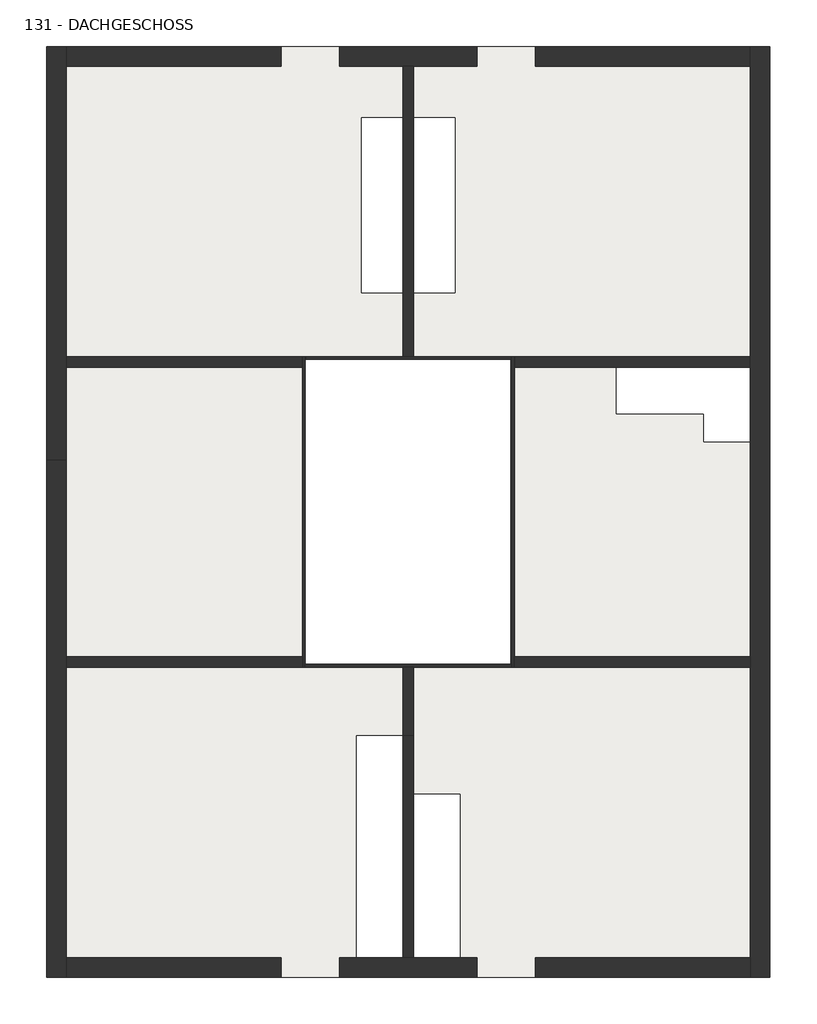
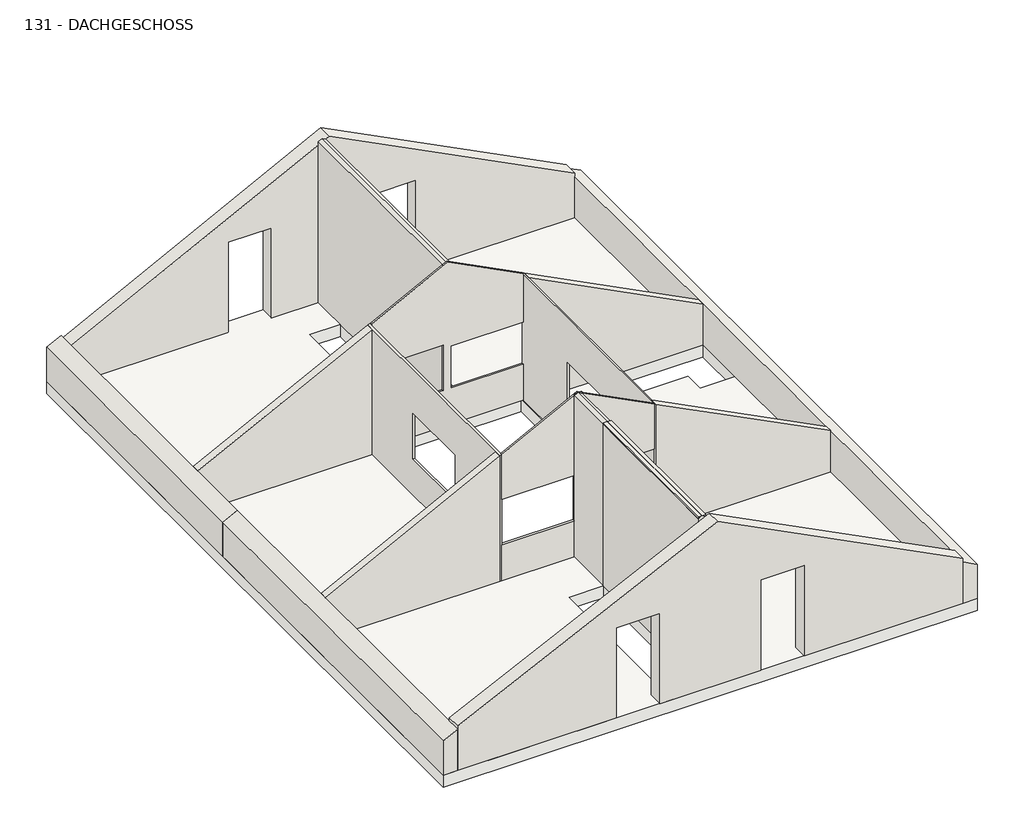
# One storey: 16 walls, 1 slab.
"""IFC4 building model written with IfcOpenShell, lengths in millimetres."""

import ifcopenshell
import ifcopenshell.guid

model = None  # the IFC model being written
_history = None  # IfcOwnerHistory: only IFC2X3 demands one
_inside = {}  # id of a spatial element -> (the spatial element, [elements in it])
_under = {}  # id of a project, library or spatial element -> (it, [spatial elements below it])
_declared = {}  # id of a project -> (the project, [libraries it declares])
_typed = {}  # id of a type object -> (the type object, [elements of that type])
_made_of = {}  # id of a material, layer set ... -> (it, [elements and type objects made of it])


def new_model(schema):
    """Start an empty IFC model of exactly this schema.

    Asked for "IFC4X3", IfcOpenShell would pick the latest addendum, in which some entities
    have other attributes; the version numbers below select the first issue.
    IFC2X3 requires an IfcOwnerHistory on every rooted entity: one is made here for all.
    """
    global model, _history
    if schema == "IFC4X3":
        model = ifcopenshell.file(schema_version=(4, 3, 0, 0))
    else:
        model = ifcopenshell.file(schema=schema)
    _inside.clear()
    _under.clear()
    _declared.clear()
    _typed.clear()
    _made_of.clear()
    _history = None
    if model.schema == "IFC2X3":
        org = make("IfcOrganization", Name="unknown")
        user = make(
            "IfcPersonAndOrganization",
            ThePerson=make("IfcPerson", FamilyName="unknown"),
            TheOrganization=org,
        )
        app = make(
            "IfcApplication",
            ApplicationDeveloper=org,
            Version="unknown",
            ApplicationFullName="unknown",
            ApplicationIdentifier="unknown",
        )
        _history = make(
            "IfcOwnerHistory",
            OwningUser=user,
            OwningApplication=app,
            ChangeAction="ADDED",
            CreationDate=0,
        )
    return model


def make(cls, **values):
    """One entity of the class cls with the attributes given. An attribute that is None is left unset."""
    return model.create_entity(
        cls, **{name: value for name, value in values.items() if value is not None}
    )


def rooted(cls, **values):
    """An entity with a GlobalId (a new one), such as an element, a storey or a relation."""
    return make(cls, GlobalId=ifcopenshell.guid.new(), OwnerHistory=_history, **values)


def si_unit(unit_type, name, prefix=None):
    """IfcSIUnit, for example si_unit("LENGTHUNIT", "METRE", prefix="MILLI")."""
    return make("IfcSIUnit", UnitType=unit_type, Prefix=prefix, Name=name)


def assignment(units):
    """IfcUnitAssignment: the units of a project."""
    return None if units is None else make("IfcUnitAssignment", Units=units)


def point(xyz):
    """IfcCartesianPoint."""
    return None if xyz is None else make("IfcCartesianPoint", Coordinates=xyz)


def direction(xyz):
    """IfcDirection."""
    return None if xyz is None else make("IfcDirection", DirectionRatios=xyz)


def frame(location, z_axis=None, x_axis=None):
    """IfcAxis2Placement3D, a coordinate frame: its origin and axes. An axis left out is left unset."""
    return make(
        "IfcAxis2Placement3D",
        Location=point(location),
        Axis=direction(z_axis),
        RefDirection=direction(x_axis),
    )


def origin():
    """The frame at (0, 0, 0) with its axes left unset."""
    return frame((0.0, 0.0, 0.0))


def place(relative_to, where):
    """IfcLocalPlacement: puts the frame where relative to a parent placement (None: the world)."""
    return make(
        "IfcLocalPlacement", PlacementRelTo=relative_to, RelativePlacement=where
    )


def context(
    kind, dimensions, precision=None, world=None, true_north=None, identifier=None
):
    """IfcGeometricRepresentationContext, for example the 3D "Model" context."""
    return make(
        "IfcGeometricRepresentationContext",
        ContextIdentifier=identifier,
        ContextType=kind,
        CoordinateSpaceDimension=dimensions,
        Precision=precision,
        WorldCoordinateSystem=world,
        TrueNorth=true_north,
    )


def project(units=None, contexts=None):
    """IfcProject with its units and contexts."""
    return rooted(
        "IfcProject",
        Name="project",
        RepresentationContexts=contexts,
        UnitsInContext=assignment(units),
    )


def spatial(cls, under=None, at=None, **own):
    """A site, building, storey or space (cls), placed at a placement, below another one or the project."""
    s = rooted(cls, ObjectPlacement=at, **own)
    if under is not None:
        _under.setdefault(under.id(), (under, []))[1].append(s)
    return s


def polyline(points):
    """IfcPolyline through the points."""
    return make("IfcPolyline", Points=[point(p) for p in points])


def outline(outer, holes=None, kind="AREA"):
    """IfcArbitraryClosedProfileDef: a profile drawn as a closed curve; with holes, ...WithVoids."""
    if holes is None:
        return make("IfcArbitraryClosedProfileDef", ProfileType=kind, OuterCurve=outer)
    return make(
        "IfcArbitraryProfileDefWithVoids",
        ProfileType=kind,
        OuterCurve=outer,
        InnerCurves=holes,
    )


def extrude(swept, where, along, depth):
    """IfcExtrudedAreaSolid: the profile swept, set in the frame where, extruded along a direction by depth."""
    return make(
        "IfcExtrudedAreaSolid",
        SweptArea=swept,
        Position=where,
        ExtrudedDirection=direction(along),
        Depth=depth,
    )


def faces_of(points, faces, orient=None, outer=None):
    """IfcFace entities. A face is a list of loops; a loop is a list of indices into points, from 0.

    orient and outer hold one flag for each loop. By default every Orientation is true, the
    first loop of a face is its IfcFaceOuterBound and the others are IfcFaceBound.
    """
    made = []
    for i, loops in enumerate(faces):
        bounds = []
        for j, loop in enumerate(loops):
            is_outer = j == 0 if outer is None else outer[i][j]
            bounds.append(
                make(
                    "IfcFaceOuterBound" if is_outer else "IfcFaceBound",
                    Bound=make("IfcPolyLoop", Polygon=[points[k] for k in loop]),
                    Orientation=True if orient is None else orient[i][j],
                )
            )
        made.append(make("IfcFace", Bounds=bounds))
    return made


def faceted_brep(points, faces, orient=None, outer=None, voids=None):
    """IfcFacetedBrep: a solid bounded by flat faces; with voids (closed shells), ...WithVoids."""
    shared = [point(p) for p in points]
    hull = make("IfcClosedShell", CfsFaces=faces_of(shared, faces, orient, outer))
    if voids is None:
        return make("IfcFacetedBrep", Outer=hull)
    return make(
        "IfcFacetedBrepWithVoids",
        Outer=hull,
        Voids=[
            make(cls, CfsFaces=faces_of(shared, fs, o, b)) for cls, fs, o, b in voids
        ],
    )


def shape(context_of_items, identifier, shape_type, items):
    """IfcShapeRepresentation: the items that make up one representation, for example the "Body"."""
    return make(
        "IfcShapeRepresentation",
        ContextOfItems=context_of_items,
        RepresentationIdentifier=identifier,
        RepresentationType=shape_type,
        Items=items,
    )


def source(mapping_origin, context_of_items, identifier, shape_type, items):
    """IfcRepresentationMap: a shape defined once, which mapped items show again and again."""
    return make(
        "IfcRepresentationMap",
        MappingOrigin=mapping_origin,
        MappedRepresentation=shape(context_of_items, identifier, shape_type, items),
    )


def transform(
    local_origin,
    x_axis=None,
    y_axis=None,
    z_axis=None,
    scale=None,
    scale2=None,
    scale3=None,
    uniform=True,
):
    """IfcCartesianTransformationOperator3D, or its non-uniform kind. x_axis, y_axis, z_axis: its Axis1, 2, 3."""
    if uniform:
        return make(
            "IfcCartesianTransformationOperator3D",
            Axis1=direction(x_axis),
            Axis2=direction(y_axis),
            LocalOrigin=point(local_origin),
            Scale=scale,
            Axis3=direction(z_axis),
        )
    return make(
        "IfcCartesianTransformationOperator3DnonUniform",
        Axis1=direction(x_axis),
        Axis2=direction(y_axis),
        LocalOrigin=point(local_origin),
        Scale=scale,
        Axis3=direction(z_axis),
        Scale2=scale2,
        Scale3=scale3,
    )


def mapped(mapping_source, mapping_target):
    """IfcMappedItem: shows the shape of a source again, moved by a transform."""
    return make(
        "IfcMappedItem", MappingSource=mapping_source, MappingTarget=mapping_target
    )


def made_of(thing, what):
    """Note that an element or type object is made of a material, layer set ...; save() writes the relation."""
    if what is not None:
        _made_of.setdefault(what.id(), (what, []))[1].append(thing)
    return thing


def element(
    cls,
    number,
    at=None,
    inside=None,
    cuts=None,
    type_object=None,
    material=None,
    context=None,
    identifier="Body",
    shape_type=None,
    held_by="IfcProductDefinitionShape",
    body=None,
    shapes=None,
    **own,
):
    """One element of the class cls, such as IfcWall. Its Tag is "e" and its number.

    at: its placement. inside: the storey or other place that contains it. cuts: it is an
    opening in that element (IfcRelVoidsElement). A single representation is given by context,
    identifier, shape_type and body (its items); several are given by shapes. held_by: the class
    of the entity that holds the representations. save() writes the other relations.
    """
    e = rooted(cls, Tag="e%d" % number, ObjectPlacement=at, **own)
    if body is not None:
        shapes = [shape(context, identifier, shape_type, body)]
    if shapes is not None:
        e.Representation = make(held_by, Representations=shapes)
    if inside is not None:
        _inside.setdefault(inside.id(), (inside, []))[1].append(e)
    if cuts is not None:
        rooted(
            "IfcRelVoidsElement", RelatingBuildingElement=cuts, RelatedOpeningElement=e
        )
    if type_object is not None:
        _typed.setdefault(type_object.id(), (type_object, []))[1].append(e)
    return made_of(e, material)


def aggregate(whole, parts):
    """IfcRelAggregates: a whole, such as a stair, and the parts it consists of."""
    return rooted("IfcRelAggregates", RelatingObject=whole, RelatedObjects=parts)


def save(model, path):
    """Write the relations noted so far, then the file.

    IfcRelAggregates (storeys below a building ...), IfcRelContainedInSpatialStructure (elements
    in a storey), IfcRelDefinesByType, IfcRelAssociatesMaterial and IfcRelDeclares: one each for
    every whole, place, type object, material and project.
    """
    for whole, parts in _under.values():
        aggregate(whole, parts)
    for where, things in _inside.values():
        rooted(
            "IfcRelContainedInSpatialStructure",
            RelatedElements=things,
            RelatingStructure=where,
        )
    for kind, things in _typed.values():
        rooted("IfcRelDefinesByType", RelatedObjects=things, RelatingType=kind)
    for what, things in _made_of.values():
        rooted("IfcRelAssociatesMaterial", RelatedObjects=things, RelatingMaterial=what)
    for by, libraries in _declared.values():
        rooted("IfcRelDeclares", RelatingContext=by, RelatedDefinitions=libraries)
    model.write(path)


def slab_52cff1b9(model_context):
    return source(origin(), model_context, "Body", "SweptSolid", [
        extrude(outline(polyline([(172797.7593015, 28481.9343946), (158797.7593015, 28481.9343946), (158797.7593015, 46484.7962965), (172797.7593015, 46484.7962965), (172797.7593015, 28481.9343946)]), holes=[polyline([(167772.7593015, 40484.7962965), (163772.7593015, 40484.7962965), (163772.7593015, 34484.7962965), (167772.7593015, 34484.7962965), (167772.7593015, 40484.7962965)]), polyline([(165697.7593015, 33159.7962965), (164797.7593015, 33159.7962965), (164797.7593015, 28861.9343946), (165697.7593015, 28861.9343946), (165697.7593015, 33159.7962965)]), polyline([(165897.7593015, 32021.9343946), (165897.7593015, 29779.7962965), (165897.7593015, 28861.9343946), (166797.7593015, 28861.9343946), (166797.7593015, 32021.9343946), (165897.7593015, 32021.9343946)]), polyline([(171517.7593015, 38844.7962965), (172417.7593015, 38844.7962965), (172417.7593015, 40284.7962965), (169822.7593015, 40284.7962965), (169822.7593015, 39384.7962965), (171517.7593015, 39384.7962965), (171517.7593015, 38844.7962965)]), polyline([(165897.7593015, 45104.7962965), (165897.7593015, 41724.7962965), (166697.7593015, 41724.7962965), (166697.7593015, 45104.7962965), (165897.7593015, 45104.7962965)]), polyline([(164897.7593015, 41724.7962965), (165697.7593015, 41724.7962965), (165697.7593015, 45104.7962965), (164897.7593015, 45104.7962965), (164897.7593015, 41724.7962965)])]), frame((0.0, 0.0, 5830.0), z_axis=(0.0, 0.0, 1.0), x_axis=(1.0, 0.0, 0.0)), (0.0, 0.0, 1.0), 330.0),
    ])


model = new_model("IFC4")

# Units and contexts
model_context = context("Model", 3, world=origin())
ifc_project = project(units=[si_unit("LENGTHUNIT", "METRE", prefix="MILLI")], contexts=[model_context])

# Site, building, storey
site = spatial("IfcSite", under=ifc_project)
building = spatial("IfcBuilding", under=site)
storey = spatial("IfcBuildingStorey", under=building, Name="131 - DACHGESCHOSS", Elevation=5650.0)

# Slab
placement = place(None, origin())
slab_shape = slab_52cff1b9(model_context)
element("IfcSlab", 1, ObjectType="Holzdecke 142136 : Holzdecke 142136", at=placement, inside=storey, context=model_context, shape_type="MappedRepresentation", body=[
    mapped(slab_shape, transform((-157297.7593015, -26934.7962965, 0.0), x_axis=(1.0, 0.0, 0.0), y_axis=(0.0, 1.0, 0.0), z_axis=(0.0, 0.0, 1.0))),
])

# Walls
element("IfcWall", 2, ObjectType="Holzwand", at=placement, inside=storey, context=model_context, shape_type="SweptSolid", body=[
    extrude(outline(polyline([(6160.0, 10550.0), (6160.0, 15120.0), (7303.6196708, 15120.0), (9632.150975, 10550.0), (6160.0, 10550.0)])), frame((0.0, 7550.0, 0.0), z_axis=(0.0, 1.0, 0.0), x_axis=(0.0, 0.0, 1.0)), (0.0, 0.0, 1.0), 200.0),
])
element("IfcWall", 3, ObjectType="Holzwand:1197", at=placement, inside=storey, context=model_context, shape_type="SweptSolid", body=[
    extrude(outline(polyline([(6160.0, 1880.0), (6160.0, 6450.0), (9632.150975, 6450.0), (7303.6196708, 1880.0), (6160.0, 1880.0)])), frame((0.0, 7550.0, 0.0), z_axis=(0.0, 1.0, 0.0), x_axis=(0.0, 0.0, 1.0)), (0.0, 0.0, 1.0), 200.0),
])
element("IfcWall", 4, ObjectType="Holzwand:1195", at=placement, inside=storey, context=model_context, shape_type="SweptSolid", body=[
    extrude(outline(polyline([(6160.0, 10550.0), (6160.0, 15120.0), (7303.6196708, 15120.0), (9632.150975, 10550.0), (6160.0, 10550.0)])), frame((0.0, 13350.0, 0.0), z_axis=(0.0, 1.0, 0.0), x_axis=(0.0, 0.0, 1.0)), (0.0, 0.0, 1.0), 200.0),
])
element("IfcWall", 5, ObjectType="Holzwand:1193", at=placement, inside=storey, context=model_context, shape_type="SweptSolid", body=[
    extrude(outline(polyline([(6160.0, 1880.0), (6160.0, 6450.0), (9632.150975, 6450.0), (7303.6196708, 1880.0), (6160.0, 1880.0)])), frame((0.0, 13350.0, 0.0), z_axis=(0.0, 1.0, 0.0), x_axis=(0.0, 0.0, 1.0)), (0.0, 0.0, 1.0), 200.0),
])
element("IfcWall", 6, ObjectType=" ", at=placement, inside=storey, context=model_context, shape_type="Brep", body=[
    faceted_brep([(6500.0, 7550.0, 6160.0), (6500.0, 7600.0, 6160.0), (6500.0, 13550.0, 6160.0), (6500.0, 13550.0, 9657.6272475), (6500.0, 7600.0, 9657.6272475), (6500.0, 7550.0, 9657.6272475), (6500.0, 7550.0, 8420.0), (6500.0, 7550.0, 7160.0), (6500.0, 11500.0, 8420.0), (6500.0, 11500.0, 7160.0), (6500.0, 9600.0, 7160.0), (6500.0, 9600.0, 8420.0), (6450.0, 13550.0, 6160.0), (6450.0, 7550.0, 6160.0), (6450.0, 7550.0, 9632.150975), (6450.0, 13550.0, 9632.150975), (6450.0, 11500.0, 7160.0), (6450.0, 11500.0, 8420.0), (6450.0, 9600.0, 8420.0), (6450.0, 9600.0, 7160.0)], [[[0, 1, 2, 3, 4, 5, 6, 7], [8, 9, 10, 11]], [[12, 13, 14, 15], [16, 17, 18, 19]], [[2, 1, 0, 13, 12]], [[5, 4, 3, 15, 14]], [[8, 17, 16, 9]], [[17, 8, 11, 18]], [[18, 11, 10, 19]], [[9, 16, 19, 10]], [[0, 7, 6, 5, 14, 13]], [[3, 2, 12, 15]]]),
])
element("IfcWall", 7, ObjectType=" :1188", at=placement, inside=storey, context=model_context, shape_type="Brep", body=[
    faceted_brep([(10500.0, 7600.0, 6160.0), (6500.0, 7600.0, 6160.0), (6500.0, 7600.0, 7160.0), (8400.0, 7600.0, 7160.0), (8400.0, 7600.0, 8420.0), (6500.0, 7600.0, 8420.0), (6500.0, 7600.0, 9657.6272475), (8500.0, 7600.0, 10676.6781465), (10500.0, 7600.0, 9657.6272475), (10500.0, 7600.0, 8420.0), (8607.9636779, 7600.0, 8420.0), (8607.9636779, 7600.0, 7160.0), (10500.0, 7600.0, 7160.0), (6500.0, 7550.0, 6160.0), (10500.0, 7550.0, 6160.0), (10500.0, 7550.0, 7160.0), (8607.9636779, 7550.0, 7160.0), (8607.9636779, 7550.0, 8420.0), (10500.0, 7550.0, 8420.0), (10500.0, 7550.0, 9657.6272475), (8600.0, 7550.0, 10625.7256015), (8600.0, 7550.0, 10676.6781465), (8400.0, 7550.0, 10676.6781465), (8400.0, 7550.0, 10625.7256015), (6500.0, 7550.0, 9657.6272475), (6500.0, 7550.0, 8420.0), (8400.0, 7550.0, 8420.0), (8400.0, 7550.0, 7160.0), (6500.0, 7550.0, 7160.0), (8500.0, 7550.4030929, 10676.6781465)], [[[0, 1, 2, 3, 4, 5, 6, 7, 8, 9, 10, 11, 12]], [[13, 14, 15, 16, 17, 18, 19, 20, 21, 22, 23, 24, 25, 26, 27, 28]], [[1, 0, 14, 13]], [[22, 21, 29]], [[29, 20, 19, 8, 7]], [[20, 29, 21]], [[29, 7, 6, 24, 23]], [[29, 23, 22]], [[4, 26, 25, 5]], [[26, 4, 3, 27]], [[27, 3, 2, 28]], [[10, 17, 16, 11]], [[17, 10, 9, 18]], [[11, 16, 15, 12]], [[8, 19, 18, 9]], [[14, 0, 12, 15]], [[24, 6, 5, 25]], [[1, 13, 28, 2]]]),
])
element("IfcWall", 8, ObjectType=" :1186", at=placement, inside=storey, context=model_context, shape_type="Brep", body=[
    faceted_brep([(10500.0, 13550.0, 6160.0), (10500.0, 13500.0, 6160.0), (10500.0, 7600.0, 6160.0), (10500.0, 7550.0, 6160.0), (10500.0, 7550.0, 7160.0), (10500.0, 7550.0, 8420.0), (10500.0, 7550.0, 9657.6272475), (10500.0, 7600.0, 9657.6272475), (10500.0, 13550.0, 9657.6272475), (10500.0, 13550.0, 8320.0), (10500.0, 13550.0, 7160.0), (10500.0, 9600.0, 8420.0), (10500.0, 9600.0, 7160.0), (10500.0, 11500.0, 7160.0), (10500.0, 11500.0, 8420.0), (10550.0, 7550.0, 6160.0), (10550.0, 13550.0, 6160.0), (10550.0, 13550.0, 9632.150975), (10550.0, 7550.0, 9632.150975), (10550.0, 9600.0, 7160.0), (10550.0, 9600.0, 8420.0), (10550.0, 11500.0, 8420.0), (10550.0, 11500.0, 7160.0)], [[[0, 1, 2, 3, 4, 5, 6, 7, 8, 9, 10], [11, 12, 13, 14]], [[15, 16, 17, 18], [19, 20, 21, 22]], [[3, 2, 1, 0, 16, 15]], [[8, 7, 6, 18, 17]], [[19, 12, 11, 20]], [[20, 11, 14, 21]], [[21, 14, 13, 22]], [[12, 19, 22, 13]], [[6, 5, 4, 3, 15, 18]], [[0, 10, 9, 8, 17, 16]]]),
])
element("IfcWall", 9, ObjectType="Holzwand:1184", at=placement, inside=storey, context=model_context, shape_type="SweptSolid", body=[
    extrude(outline(polyline([(6160.0, 8400.0), (6160.0, 8600.0), (10625.7256015, 8600.0), (10676.6781465, 8500.0), (10625.7256015, 8400.0), (6160.0, 8400.0)])), frame((0.0, 1927.1380981, 0.0), z_axis=(0.0, 1.0, 0.0), x_axis=(0.0, 0.0, 1.0)), (0.0, 0.0, 1.0), 4297.8619019),
])
element("IfcWall", 10, ObjectType=" :1182", at=placement, inside=storey, context=model_context, shape_type="Brep", body=[
    faceted_brep([(1880.0, 1547.1380981, 6160.0), (1880.0, 1927.1380981, 6160.0), (1880.0, 11550.0, 6160.0), (1880.0, 11550.0, 7303.6196708), (1880.0, 1547.1380981, 7303.6196708), (1500.0, 11550.0, 6160.0), (1500.0, 1547.1380981, 6160.0), (1500.0, 1547.1380981, 7110.0), (1500.0, 11550.0, 7110.0)], [[[0, 1, 2, 3, 4]], [[5, 6, 7, 8]], [[2, 1, 0, 6, 5]], [[3, 2, 5, 8]], [[4, 3, 8, 7]], [[0, 4, 7, 6]]]),
])
element("IfcWall", 11, ObjectType="Holzwand:1180", at=placement, inside=storey, context=model_context, shape_type="SweptSolid", body=[
    extrude(outline(polyline([(6160.0, 8400.0), (6160.0, 8600.0), (10625.7256015, 8600.0), (10676.6781465, 8500.0), (10625.7256015, 8400.0), (6160.0, 8400.0)])), frame((0.0, 13550.0, 0.0), z_axis=(0.0, 1.0, 0.0), x_axis=(0.0, 0.0, 1.0)), (0.0, 0.0, 1.0), 5620.0),
])
element("IfcWall", 12, ObjectType="Holzwand:1178", at=placement, inside=storey, context=model_context, shape_type="Brep", body=[
    faceted_brep([(8600.0, 1927.541191, 6160.0), (8600.0, 7550.0, 6160.0), (8600.0, 7550.0, 10625.7256015), (8600.0, 6225.0, 10625.7256015), (8600.0, 6225.0, 10676.6781465), (8600.0, 1927.541191, 10676.6781465), (8400.0, 7550.0, 6160.0), (8400.0, 1927.541191, 6160.0), (8400.0, 1927.541191, 10676.6781465), (8400.0, 6225.0, 10676.6781465), (8400.0, 6225.0, 10625.7256015), (8400.0, 7550.0, 10625.7256015), (8500.0, 6225.0, 10676.6781465), (8500.0, 7550.0, 10676.6781465)], [[[0, 1, 2, 3, 4, 5]], [[6, 7, 8, 9, 10, 11]], [[1, 0, 7, 6]], [[8, 5, 4, 12, 9]], [[0, 5, 8, 7]], [[12, 3, 2, 13]], [[3, 12, 4]], [[12, 10, 9]], [[10, 12, 13, 11]], [[1, 6, 11, 13, 2]]]),
])
element("IfcWall", 13, ObjectType=" :1176", at=placement, inside=storey, context=model_context, shape_type="Brep", body=[
    faceted_brep([(15120.0, 19550.0, 6160.0), (15120.0, 19170.0, 6160.0), (15120.0, 1927.1380981, 6160.0), (15120.0, 1547.1380981, 6160.0), (15120.0, 1547.1380981, 7303.6196708), (15120.0, 19550.0, 7303.6196708), (15500.0, 1547.1380981, 6160.0), (15500.0, 19550.0, 6160.0), (15500.0, 19550.0, 7110.0), (15500.0, 1547.1380981, 7110.0)], [[[0, 1, 2, 3, 4, 5]], [[6, 7, 8, 9]], [[3, 2, 1, 0, 7, 6]], [[5, 4, 9, 8]], [[4, 3, 6, 9]], [[0, 5, 8, 7]]]),
])
element("IfcWall", 14, ObjectType=" :1174", at=placement, inside=storey, context=model_context, shape_type="Brep", body=[
    faceted_brep([(1880.0, 11550.0, 6160.0), (1880.0, 19170.0, 6160.0), (1880.0, 19550.0, 6160.0), (1880.0, 19550.0, 7206.8098354), (1880.0, 19550.0, 7303.6196708), (1880.0, 11550.0, 7303.6196708), (1500.0, 19550.0, 6160.0), (1500.0, 11550.0, 6160.0), (1500.0, 11550.0, 7110.0), (1500.0, 19550.0, 7110.0)], [[[0, 1, 2, 3, 4, 5]], [[6, 7, 8, 9]], [[2, 1, 0, 7, 6]], [[0, 5, 8, 7]], [[5, 4, 9, 8]], [[4, 3, 2, 6, 9]]]),
])
element("IfcWall", 15, ObjectType=" :1190", at=placement, inside=storey, context=model_context, shape_type="Brep", body=[
    faceted_brep([(6525.0, 13500.0, 6160.0), (10500.0, 13500.0, 6160.0), (10500.0, 13500.0, 7160.0), (8600.0, 13500.0, 7160.0), (8600.0, 13500.0, 8320.0), (10500.0, 13500.0, 8320.0), (10500.0, 13500.0, 9670.3653837), (8525.0, 13500.0, 10676.6781465), (6525.0, 13500.0, 9657.6272475), (6525.0, 13500.0, 8420.0), (8400.0, 13500.0, 8420.0), (8400.0, 13500.0, 7160.0), (6525.0, 13500.0, 7160.0), (10500.0, 13550.0, 6160.0), (6525.0, 13550.0, 6160.0), (6525.0, 13550.0, 7160.0), (8400.0, 13550.0, 7160.0), (8400.0, 13550.0, 8420.0), (6525.0, 13550.0, 8420.0), (6525.0, 13550.0, 9657.6272475), (8525.0, 13550.0, 10676.6781465), (10500.0, 13550.0, 9670.3653837), (10500.0, 13550.0, 9657.6272475), (10500.0, 13550.0, 8320.0), (8600.0, 13550.0, 8320.0), (8600.0, 13550.0, 7160.0), (10500.0, 13550.0, 7160.0)], [[[0, 1, 2, 3, 4, 5, 6, 7, 8, 9, 10, 11, 12]], [[13, 14, 15, 16, 17, 18, 19, 20, 21, 22, 23, 24, 25, 26]], [[1, 0, 14, 13]], [[7, 6, 21, 20]], [[8, 7, 20, 19]], [[8, 19, 18, 9]], [[14, 0, 12, 15]], [[10, 17, 16, 11]], [[17, 10, 9, 18]], [[11, 16, 15, 12]], [[4, 24, 23, 5]], [[24, 4, 3, 25]], [[25, 3, 2, 26]], [[21, 6, 5, 23, 22]], [[1, 13, 26, 2]]]),
])
element("IfcWall", 16, ObjectType=" :1201", at=placement, inside=storey, context=model_context, shape_type="Brep", body=[
    faceted_brep([(1880.0, 1927.1380981, 7395.1741151), (8690.0, 1927.1380981, 10676.6781465), (15120.0, 1927.1380981, 7400.4295062), (15120.0, 1927.1380981, 6160.0), (10960.0, 1927.1380981, 6160.0), (10960.0, 1927.1380981, 8660.0), (9825.0, 1927.1380981, 8660.0), (9825.0, 1927.1380981, 6160.0), (7175.0, 1927.1380981, 6160.0), (7175.0, 1927.1380981, 8660.0), (6040.0, 1927.1380981, 8660.0), (6040.0, 1927.1380981, 6160.0), (1880.0, 1927.1380981, 6160.0), (8690.0, 1547.1380981, 10676.6781465), (1880.0, 1547.1380981, 7395.1741151), (1880.0, 1547.1380981, 7303.6196708), (1880.0, 1547.1380981, 6160.0), (6040.0, 1547.1380981, 6160.0), (6040.0, 1547.1380981, 8660.0), (7175.0, 1547.1380981, 8660.0), (7175.0, 1547.1380981, 6160.0), (9825.0, 1547.1380981, 6160.0), (9825.0, 1547.1380981, 8660.0), (10960.0, 1547.1380981, 8660.0), (10960.0, 1547.1380981, 6160.0), (15120.0, 1547.1380981, 6160.0), (15120.0, 1547.1380981, 7303.6196708), (15120.0, 1547.1380981, 7400.4295062)], [[[0, 1, 2, 3, 4, 5, 6, 7, 8, 9, 10, 11, 12]], [[13, 14, 15, 16, 17, 18, 19, 20, 21, 22, 23, 24, 25, 26, 27]], [[4, 3, 25, 24]], [[7, 21, 20, 8]], [[16, 12, 11, 17]], [[1, 0, 14, 13]], [[2, 1, 13, 27]], [[23, 5, 4, 24]], [[5, 23, 22, 6]], [[6, 22, 21, 7]], [[19, 9, 8, 20]], [[9, 19, 18, 10]], [[10, 18, 17, 11]], [[0, 12, 16, 15, 14]], [[3, 2, 27, 26, 25]]]),
])
element("IfcWall", 17, ObjectType=" :1202", at=placement, inside=storey, context=model_context, shape_type="Brep", body=[
    faceted_brep([(15120.0, 19170.0, 7400.4295062), (8690.0, 19170.0, 10676.6781465), (1880.0, 19170.0, 7206.8098354), (1880.0, 19170.0, 6160.0), (6040.0, 19170.0, 6160.0), (6040.0, 19170.0, 8660.0), (7175.0, 19170.0, 8660.0), (7175.0, 19170.0, 6160.0), (9825.0, 19170.0, 6160.0), (9825.0, 19170.0, 8660.0), (10960.0, 19170.0, 8660.0), (10960.0, 19170.0, 6160.0), (15120.0, 19170.0, 6160.0), (8690.0, 19550.0, 10676.6781465), (15120.0, 19550.0, 7400.4295062), (15120.0, 19550.0, 7303.6196708), (15120.0, 19550.0, 6160.0), (10960.0, 19550.0, 6160.0), (10960.0, 19550.0, 8660.0), (9825.0, 19550.0, 8660.0), (9825.0, 19550.0, 6160.0), (7175.0, 19550.0, 6160.0), (7175.0, 19550.0, 8660.0), (6040.0, 19550.0, 8660.0), (6040.0, 19550.0, 6160.0), (1880.0, 19550.0, 6160.0), (1880.0, 19550.0, 7206.8098354)], [[[0, 1, 2, 3, 4, 5, 6, 7, 8, 9, 10, 11, 12]], [[13, 14, 15, 16, 17, 18, 19, 20, 21, 22, 23, 24, 25, 26]], [[12, 11, 17, 16]], [[20, 8, 7, 21]], [[3, 25, 24, 4]], [[1, 0, 14, 13]], [[2, 1, 13, 26]], [[19, 9, 8, 20]], [[9, 19, 18, 10]], [[10, 18, 17, 11]], [[23, 5, 4, 24]], [[5, 23, 22, 6]], [[6, 22, 21, 7]], [[0, 12, 16, 15, 14]], [[3, 2, 26, 25]]]),
])

save(model, "model.ifc")

# Revit data of these elements
# Type "Holzdecke 142136 : Holzdecke 142136"
#   Abrechnungsart = "m²"
#   Allright_Bauteil_ID = "0123De 0783954319"
#   Bezeichnung = "Holzdecke"
#   Codetext = "D-HOLZBALKEN1\\"
#   Gewerk = "Zimmer- und Holzbauarbeiten"
#   Material = "Holz"
#   Objektname = "Brettstapeldecke"
#   NameOverride = "Holzdecke"
#   Reference = "Holzdecke"
#   Status = "NEW"
#   PitchAngle = 0.00°
#   ThermalTransmittance = 0.0000 BTU/(h·ft²·°F)
#   2D Interaktion = yes
#   Combustible = no
#   Compartmentation = no
#   IsExternal = no
#   LoadBearing = yes
# Type "Holzwand"
#   ThermalTransmittance = 0.0000 BTU/(h·ft²·°F)
#   Combustible = no
#   Compartmentation = no
#   Layers, outside or top first: 0.200 m "holzschalung" (function 1)
# Type "Holzwand:1197"
#   ThermalTransmittance = 0.0000 BTU/(h·ft²·°F)
#   Combustible = no
#   Compartmentation = no
#   Layers, outside or top first: 0.200 m "holzschalung" (function 1)
# Type "Holzwand:1195"
#   ThermalTransmittance = 0.0000 BTU/(h·ft²·°F)
#   Combustible = no
#   Compartmentation = no
#   Layers, outside or top first: 0.200 m "holzschalung" (function 1)
# Type "Holzwand:1193"
#   ThermalTransmittance = 0.0000 BTU/(h·ft²·°F)
#   Combustible = no
#   Compartmentation = no
#   Layers, outside or top first: 0.200 m "holzschalung" (function 1)
# Type " "
#   Layers, outside or top first: 0.050 m "holzschalung" (function 1)
# Type " :1188"
#   Layers, outside or top first: 0.050 m "holzschalung" (function 1)
# Type " :1186"
#   Layers, outside or top first: 0.050 m "holzschalung" (function 1)
# Type "Holzwand:1184"
#   ThermalTransmittance = 0.0000 BTU/(h·ft²·°F)
#   Combustible = no
#   Compartmentation = no
#   Layers, outside or top first: 0.200 m "holzschalung" (function 1)
# Type " :1182"
#   Layers, outside or top first: 0.380 m "holzschalung" (function 1)
# Type "Holzwand:1180"
#   ThermalTransmittance = 0.0000 BTU/(h·ft²·°F)
#   Combustible = no
#   Compartmentation = no
#   Layers, outside or top first: 0.200 m "holzschalung" (function 1)
# Type "Holzwand:1178"
#   ThermalTransmittance = 0.0000 BTU/(h·ft²·°F)
#   Combustible = no
#   Compartmentation = no
#   Layers, outside or top first: 0.200 m "holzschalung" (function 1)
# Type " :1176"
#   Layers, outside or top first: 0.380 m "holzschalung" (function 1)
# Type " :1174"
#   Layers, outside or top first: 0.380 m "holzschalung" (function 1)
# Type " :1190"
#   Layers, outside or top first: 0.050 m "holzschalung" (function 1)
# Type " :1201"
#   Layers, outside or top first: 0.380 m "holzschalung" (function 1)
# Type " :1202"
#   Layers, outside or top first: 0.380 m "holzschalung" (function 1)
# Element 1 (IfcSlab, "Holzdecke 142136 : Holzdecke 142136")
#   IFC Predefined Type = "FLOOR"
#   Export to IFC As = "ifcslab"
#   IfcGUID = "2UFX_hum15ZQP8rfQ2hTBa"
#   Phase Created = New Construction
#   Materials on its faces: "holzschalung"
# Element 2 (IfcWall, "Holzwand")
#   Export to IFC As = "ifcwall"
#   IfcGUID = "2irPo0fN95hwd6nGWO8xKX"
#   NameOverride = "Holzwand"
#   Abrechnungsart = "St"
#   Allright_Bauteil_ID = "0131HWa0658953274"
#   Bezeichnung = "Holzwand"
#   Layer #1:Object Layer Attributes #1:Abrechnungsart = "m²"
#   Layer #1:Object Layer Attributes #1:Allright_Bauteil_ID = "0131Wa 0658953275"
#   Layer #1:Object Layer Attributes #1:Bezeichnung = "Holzwand"
#   Layer #1:Object Layer Attributes #1:Codetext = "HO-WI-HSW\\"
#   Layer #1:Object Layer Attributes #1:Gewerk = "Zimmer- und Holzbauarbeiten"
#   Layer #1:Object Layer Attributes #1:Material = "Holz"
#   Layer #1:Object Layer Attributes #1:Objektname = "Wand"
#   Layer #1:Object Layer Attributes #1:Reference = "Holzwand"
#   Layer #1:Object Layer Attributes #1:Status = "Neubau"
#   MEP Wandtyp = "HO-WA-HSW\\"
#   Objektname = "Gesamtwand"
#   Reference = "Holzwand"
#   Status = "NEW"
#   built-in parameter 1001111 = 0.510 m
#   Top Offset = 0.000 m
#   Base Offset = 0.510 m
#   Unconnected Height = 3.497627 m
#   wall height = 3.497627 m
#   Layer #1:Object Layer Attributes #1:U-Wert = 0
#   Layer #1:Object Layer Attributes #1:2D Interaktion = yes
#   Layer #1:Object Layer Attributes #1:Außenbauteil = no
#   Layer #1:Object Layer Attributes #1:Brandabschnittsdefinierendes Bauteil = no
#   Layer #1:Object Layer Attributes #1:Brennbares Material = no
#   Layer #1:Object Layer Attributes #1:Raumhohe Wand = yes
#   Layer #1:Object Layer Attributes #1:Tragendes Bauteil = yes
#   ExtendToStructure = yes
#   IsExternal = no
#   LoadBearing = yes
#   Phase Created = New Construction
#   Base Constraint = 131 - DACHGESCHOSS
#   Materials on its faces: "holzschalung"
# Element 3 (IfcWall, "Holzwand:1197")
#   Export to IFC As = "ifcwall"
#   IfcGUID = "0btdfUgAf1BODjBN4XyqI6"
#   NameOverride = "Holzwand"
#   Abrechnungsart = "St"
#   Allright_Bauteil_ID = "0131HWa0658955859"
#   Bezeichnung = "Holzwand"
#   Layer #1:Object Layer Attributes #1:Abrechnungsart = "m²"
#   Layer #1:Object Layer Attributes #1:Allright_Bauteil_ID = "0131Wa 0658955860"
#   Layer #1:Object Layer Attributes #1:Bezeichnung = "Holzwand"
#   Layer #1:Object Layer Attributes #1:Codetext = "HO-WI-HSW\\"
#   Layer #1:Object Layer Attributes #1:Gewerk = "Zimmer- und Holzbauarbeiten"
#   Layer #1:Object Layer Attributes #1:Material = "Holz"
#   Layer #1:Object Layer Attributes #1:Objektname = "Wand"
#   Layer #1:Object Layer Attributes #1:Reference = "Holzwand"
#   Layer #1:Object Layer Attributes #1:Status = "Neubau"
#   MEP Wandtyp = "HO-WA-HSW\\"
#   Objektname = "Gesamtwand"
#   Reference = "Holzwand"
#   Status = "NEW"
#   built-in parameter 1001111 = 0.510 m
#   Top Offset = 0.000 m
#   Base Offset = 0.510 m
#   Unconnected Height = 3.497627 m
#   wall height = 3.497627 m
#   Layer #1:Object Layer Attributes #1:U-Wert = 0
#   Layer #1:Object Layer Attributes #1:2D Interaktion = yes
#   Layer #1:Object Layer Attributes #1:Außenbauteil = no
#   Layer #1:Object Layer Attributes #1:Brandabschnittsdefinierendes Bauteil = no
#   Layer #1:Object Layer Attributes #1:Brennbares Material = no
#   Layer #1:Object Layer Attributes #1:Raumhohe Wand = yes
#   Layer #1:Object Layer Attributes #1:Tragendes Bauteil = yes
#   ExtendToStructure = yes
#   IsExternal = no
#   LoadBearing = yes
#   Phase Created = New Construction
#   Base Constraint = 131 - DACHGESCHOSS
#   Materials on its faces: "holzschalung"
# Element 4 (IfcWall, "Holzwand:1195")
#   Export to IFC As = "ifcwall"
#   IfcGUID = "2RQ2xt8jL3z9U7Ow04WNfJ"
#   NameOverride = "Holzwand"
#   Abrechnungsart = "St"
#   Allright_Bauteil_ID = "0131HWa0658953259"
#   Bezeichnung = "Holzwand"
#   Layer #1:Object Layer Attributes #1:Abrechnungsart = "m²"
#   Layer #1:Object Layer Attributes #1:Allright_Bauteil_ID = "0131Wa 0658953260"
#   Layer #1:Object Layer Attributes #1:Bezeichnung = "Holzwand"
#   Layer #1:Object Layer Attributes #1:Codetext = "HO-WI-HSW\\"
#   Layer #1:Object Layer Attributes #1:Gewerk = "Zimmer- und Holzbauarbeiten"
#   Layer #1:Object Layer Attributes #1:Material = "Holz"
#   Layer #1:Object Layer Attributes #1:Objektname = "Wand"
#   Layer #1:Object Layer Attributes #1:Reference = "Holzwand"
#   Layer #1:Object Layer Attributes #1:Status = "Neubau"
#   MEP Wandtyp = "HO-WA-HSW\\"
#   Objektname = "Gesamtwand"
#   Reference = "Holzwand"
#   Status = "NEW"
#   built-in parameter 1001111 = 0.510 m
#   Top Offset = 0.000 m
#   Base Offset = 0.510 m
#   Unconnected Height = 3.497627 m
#   wall height = 3.497627 m
#   Layer #1:Object Layer Attributes #1:U-Wert = 0
#   Layer #1:Object Layer Attributes #1:2D Interaktion = yes
#   Layer #1:Object Layer Attributes #1:Außenbauteil = no
#   Layer #1:Object Layer Attributes #1:Brandabschnittsdefinierendes Bauteil = no
#   Layer #1:Object Layer Attributes #1:Brennbares Material = no
#   Layer #1:Object Layer Attributes #1:Raumhohe Wand = yes
#   Layer #1:Object Layer Attributes #1:Tragendes Bauteil = yes
#   ExtendToStructure = yes
#   IsExternal = no
#   LoadBearing = yes
#   Phase Created = New Construction
#   Base Constraint = 131 - DACHGESCHOSS
#   Materials on its faces: "holzschalung"
# Element 5 (IfcWall, "Holzwand:1193")
#   Export to IFC As = "ifcwall"
#   IfcGUID = "1XDlXo4IT97OvdyoFppHWZ"
#   NameOverride = "Holzwand"
#   Abrechnungsart = "St"
#   Allright_Bauteil_ID = "0131HWa0658952486"
#   Bezeichnung = "Holzwand"
#   Layer #1:Object Layer Attributes #1:Abrechnungsart = "m²"
#   Layer #1:Object Layer Attributes #1:Allright_Bauteil_ID = "0131Wa 0658952490"
#   Layer #1:Object Layer Attributes #1:Bezeichnung = "Holzwand"
#   Layer #1:Object Layer Attributes #1:Codetext = "HO-WI-HSW\\"
#   Layer #1:Object Layer Attributes #1:Gewerk = "Zimmer- und Holzbauarbeiten"
#   Layer #1:Object Layer Attributes #1:Material = "Holz"
#   Layer #1:Object Layer Attributes #1:Objektname = "Wand"
#   Layer #1:Object Layer Attributes #1:Reference = "Holzwand"
#   Layer #1:Object Layer Attributes #1:Status = "Neubau"
#   MEP Wandtyp = "HO-WA-HSW\\"
#   Objektname = "Gesamtwand"
#   Reference = "Holzwand"
#   Status = "NEW"
#   built-in parameter 1001111 = 0.510 m
#   Top Offset = 0.000 m
#   Base Offset = 0.510 m
#   Unconnected Height = 3.497627 m
#   wall height = 3.497627 m
#   Layer #1:Object Layer Attributes #1:U-Wert = 0
#   Layer #1:Object Layer Attributes #1:2D Interaktion = yes
#   Layer #1:Object Layer Attributes #1:Außenbauteil = no
#   Layer #1:Object Layer Attributes #1:Brandabschnittsdefinierendes Bauteil = no
#   Layer #1:Object Layer Attributes #1:Brennbares Material = no
#   Layer #1:Object Layer Attributes #1:Raumhohe Wand = yes
#   Layer #1:Object Layer Attributes #1:Tragendes Bauteil = yes
#   ExtendToStructure = yes
#   IsExternal = no
#   LoadBearing = yes
#   Phase Created = New Construction
#   Base Constraint = 131 - DACHGESCHOSS
#   Materials on its faces: "holzschalung"
# Element 6 (IfcWall, " ")
#   Export to IFC As = "ifcwall"
#   IfcGUID = "21FF_DgHzF28s1dzPXnAcl"
#   NameOverride = " "
#   Abrechnungsart = "m³"
#   Allright_Bauteil_ID = "0131HWa0658952409"
#   Layer #1:Object Layer Attributes #1:Abrechnungsart = "m²"
#   Layer #1:Object Layer Attributes #1:Allright_Bauteil_ID = "0131Wa 0658952493"
#   Layer #1:Object Layer Attributes #1:Gewerk = "Zimmer- und Holzbauarbeiten"
#   Layer #1:Object Layer Attributes #1:Material = "k.Ausw."
#   Layer #1:Object Layer Attributes #1:Objektname = "Wand"
#   Layer #1:Object Layer Attributes #1:Status = "Neubau"
#   MEP Wandtyp = "HO-WA-HSW\\"
#   Objektname = "Gesamtwand"
#   built-in parameter 1001111 = 0.510 m
#   Top Offset = 0.000 m
#   Base Offset = 0.510 m
#   Unconnected Height = 3.497627 m
#   wall height = 3.497627 m
#   Layer #1:Object Layer Attributes #1:2D Interaktion = yes
#   Phase Created = New Construction
#   Base Constraint = 131 - DACHGESCHOSS
#   Materials on its faces: "holzschalung"
# Element 7 (IfcWall, " :1188")
#   Export to IFC As = "ifcwall"
#   IfcGUID = "1sDERupobB$8G6O8zmS_FC"
#   NameOverride = " "
#   Abrechnungsart = "m³"
#   Allright_Bauteil_ID = "0131HWa0658952407"
#   Layer #1:Object Layer Attributes #1:Abrechnungsart = "m²"
#   Layer #1:Object Layer Attributes #1:Allright_Bauteil_ID = "0131Wa 0658952497"
#   Layer #1:Object Layer Attributes #1:Gewerk = "Zimmer- und Holzbauarbeiten"
#   Layer #1:Object Layer Attributes #1:Material = "k.Ausw."
#   Layer #1:Object Layer Attributes #1:Objektname = "Wand"
#   Layer #1:Object Layer Attributes #1:Status = "Neubau"
#   MEP Wandtyp = "HO-WA-HSW\\"
#   Objektname = "Gesamtwand"
#   built-in parameter 1001111 = 0.510 m
#   Top Offset = 0.000 m
#   Base Offset = 0.510 m
#   Unconnected Height = 4.516678 m
#   wall height = 4.516678 m
#   Layer #1:Object Layer Attributes #1:2D Interaktion = yes
#   Phase Created = New Construction
#   Base Constraint = 131 - DACHGESCHOSS
#   Materials on its faces: "holzschalung"
# Element 8 (IfcWall, " :1186")
#   Export to IFC As = "ifcwall"
#   IfcGUID = "2vPa_8WInC1fLjRjt9C8qD"
#   NameOverride = " "
#   Abrechnungsart = "m³"
#   Allright_Bauteil_ID = "0131HWa0658952411"
#   Layer #1:Object Layer Attributes #1:Abrechnungsart = "m²"
#   Layer #1:Object Layer Attributes #1:Allright_Bauteil_ID = "0131Wa 0658952482"
#   Layer #1:Object Layer Attributes #1:Gewerk = "Zimmer- und Holzbauarbeiten"
#   Layer #1:Object Layer Attributes #1:Material = "k.Ausw."
#   Layer #1:Object Layer Attributes #1:Objektname = "Wand"
#   Layer #1:Object Layer Attributes #1:Status = "Neubau"
#   MEP Wandtyp = "HO-WA-HSW\\"
#   Objektname = "Gesamtwand"
#   built-in parameter 1001111 = 0.510 m
#   Top Offset = 0.000 m
#   Base Offset = 0.510 m
#   Unconnected Height = 3.497627 m
#   wall height = 3.497627 m
#   Layer #1:Object Layer Attributes #1:2D Interaktion = yes
#   Phase Created = New Construction
#   Base Constraint = 131 - DACHGESCHOSS
#   Materials on its faces: "holzschalung"
# Element 9 (IfcWall, "Holzwand:1184")
#   Export to IFC As = "ifcwall"
#   IfcGUID = "3sGwvbH0X0wRT5LbxtOghV"
#   NameOverride = "Holzwand"
#   Abrechnungsart = "St"
#   Allright_Bauteil_ID = "0131HWa0658956028"
#   Bezeichnung = "Holzwand"
#   Layer #1:Object Layer Attributes #1:Abrechnungsart = "m²"
#   Layer #1:Object Layer Attributes #1:Allright_Bauteil_ID = "0131Wa 0658956031"
#   Layer #1:Object Layer Attributes #1:Bezeichnung = "Holzwand"
#   Layer #1:Object Layer Attributes #1:Codetext = "HO-WI-HSW\\"
#   Layer #1:Object Layer Attributes #1:Gewerk = "Zimmer- und Holzbauarbeiten"
#   Layer #1:Object Layer Attributes #1:Material = "Holz"
#   Layer #1:Object Layer Attributes #1:Objektname = "Wand"
#   Layer #1:Object Layer Attributes #1:Reference = "Holzwand"
#   Layer #1:Object Layer Attributes #1:Status = "Neubau"
#   MEP Wandtyp = "HO-WA-HSW\\"
#   Objektname = "Gesamtwand"
#   Reference = "Holzwand"
#   Status = "NEW"
#   built-in parameter 1001111 = 0.510 m
#   Top Offset = 0.000 m
#   Base Offset = 0.510 m
#   Unconnected Height = 4.516678 m
#   wall height = 4.516678 m
#   Layer #1:Object Layer Attributes #1:U-Wert = 0
#   Layer #1:Object Layer Attributes #1:2D Interaktion = yes
#   Layer #1:Object Layer Attributes #1:Außenbauteil = no
#   Layer #1:Object Layer Attributes #1:Brandabschnittsdefinierendes Bauteil = no
#   Layer #1:Object Layer Attributes #1:Brennbares Material = no
#   Layer #1:Object Layer Attributes #1:Raumhohe Wand = yes
#   Layer #1:Object Layer Attributes #1:Tragendes Bauteil = yes
#   ExtendToStructure = yes
#   IsExternal = no
#   LoadBearing = yes
#   Phase Created = New Construction
#   Base Constraint = 131 - DACHGESCHOSS
#   Materials on its faces: "holzschalung"
# Element 10 (IfcWall, " :1182")
#   Export to IFC As = "ifcwall"
#   IfcGUID = "2d5_L$AAv1WBYQkgHyHFrb"
#   NameOverride = " "
#   Abrechnungsart = "m³"
#   Allright_Bauteil_ID = "0131HWa0658952452"
#   Layer #1:Object Layer Attributes #1:Abrechnungsart = "m²"
#   Layer #1:Object Layer Attributes #1:Allright_Bauteil_ID = "0131Wa 0658952457"
#   Layer #1:Object Layer Attributes #1:Gewerk = "Zimmer- und Holzbauarbeiten"
#   Layer #1:Object Layer Attributes #1:Material = "k.Ausw."
#   Layer #1:Object Layer Attributes #1:Objektname = "Wand"
#   Layer #1:Object Layer Attributes #1:Status = "Neubau"
#   MEP Wandtyp = "HO-WA-HSW\\"
#   Objektname = "Gesamtwand"
#   built-in parameter 1001111 = 0.510 m
#   Top Offset = 0.000 m
#   Base Offset = 0.510 m
#   Unconnected Height = 1.14362 m
#   wall height = 1.14362 m
#   Layer #1:Object Layer Attributes #1:2D Interaktion = yes
#   Phase Created = New Construction
#   Base Constraint = 131 - DACHGESCHOSS
#   Materials on its faces: "holzschalung"
# Element 11 (IfcWall, "Holzwand:1180")
#   Export to IFC As = "ifcwall"
#   IfcGUID = "1F6NxEW8b7hgcJafh_mgpg"
#   NameOverride = "Holzwand"
#   Abrechnungsart = "St"
#   Allright_Bauteil_ID = "0131HWa0658952466"
#   Bezeichnung = "Holzwand"
#   Layer #1:Object Layer Attributes #1:Abrechnungsart = "m²"
#   Layer #1:Object Layer Attributes #1:Allright_Bauteil_ID = "0131Wa 0658952469"
#   Layer #1:Object Layer Attributes #1:Bezeichnung = "Holzwand"
#   Layer #1:Object Layer Attributes #1:Codetext = "HO-WI-HSW\\"
#   Layer #1:Object Layer Attributes #1:Gewerk = "Zimmer- und Holzbauarbeiten"
#   Layer #1:Object Layer Attributes #1:Material = "Holz"
#   Layer #1:Object Layer Attributes #1:Objektname = "Wand"
#   Layer #1:Object Layer Attributes #1:Reference = "Holzwand"
#   Layer #1:Object Layer Attributes #1:Status = "Neubau"
#   MEP Wandtyp = "HO-WA-HSW\\"
#   Objektname = "Gesamtwand"
#   Reference = "Holzwand"
#   Status = "NEW"
#   built-in parameter 1001111 = 0.510 m
#   Top Offset = 0.000 m
#   Base Offset = 0.510 m
#   Unconnected Height = 4.516678 m
#   wall height = 4.516678 m
#   Layer #1:Object Layer Attributes #1:U-Wert = 0
#   Layer #1:Object Layer Attributes #1:2D Interaktion = yes
#   Layer #1:Object Layer Attributes #1:Außenbauteil = no
#   Layer #1:Object Layer Attributes #1:Brandabschnittsdefinierendes Bauteil = no
#   Layer #1:Object Layer Attributes #1:Brennbares Material = no
#   Layer #1:Object Layer Attributes #1:Raumhohe Wand = yes
#   Layer #1:Object Layer Attributes #1:Tragendes Bauteil = yes
#   ExtendToStructure = yes
#   IsExternal = no
#   LoadBearing = yes
#   Phase Created = New Construction
#   Base Constraint = 131 - DACHGESCHOSS
#   Materials on its faces: "holzschalung"
# Element 12 (IfcWall, "Holzwand:1178")
#   Export to IFC As = "ifcwall"
#   IfcGUID = "00NikNq3z8kAwJn0xK23rS"
#   NameOverride = "Holzwand"
#   Abrechnungsart = "St"
#   Allright_Bauteil_ID = "0131HWa0658952460"
#   Bezeichnung = "Holzwand"
#   Layer #1:Object Layer Attributes #1:Abrechnungsart = "m²"
#   Layer #1:Object Layer Attributes #1:Allright_Bauteil_ID = "0131Wa 0658952463"
#   Layer #1:Object Layer Attributes #1:Bezeichnung = "Holzwand"
#   Layer #1:Object Layer Attributes #1:Codetext = "HO-WI-HSW\\"
#   Layer #1:Object Layer Attributes #1:Gewerk = "Zimmer- und Holzbauarbeiten"
#   Layer #1:Object Layer Attributes #1:Material = "Holz"
#   Layer #1:Object Layer Attributes #1:Objektname = "Wand"
#   Layer #1:Object Layer Attributes #1:Reference = "Holzwand"
#   Layer #1:Object Layer Attributes #1:Status = "Neubau"
#   MEP Wandtyp = "HO-WA-HSW\\"
#   Objektname = "Gesamtwand"
#   Reference = "Holzwand"
#   Status = "NEW"
#   built-in parameter 1001111 = 0.510 m
#   Top Offset = 0.000 m
#   Base Offset = 0.510 m
#   Unconnected Height = 4.516678 m
#   wall height = 4.516678 m
#   Layer #1:Object Layer Attributes #1:U-Wert = 0
#   Layer #1:Object Layer Attributes #1:2D Interaktion = yes
#   Layer #1:Object Layer Attributes #1:Außenbauteil = no
#   Layer #1:Object Layer Attributes #1:Brandabschnittsdefinierendes Bauteil = no
#   Layer #1:Object Layer Attributes #1:Brennbares Material = no
#   Layer #1:Object Layer Attributes #1:Raumhohe Wand = yes
#   Layer #1:Object Layer Attributes #1:Tragendes Bauteil = yes
#   ExtendToStructure = yes
#   IsExternal = no
#   LoadBearing = yes
#   Phase Created = New Construction
#   Base Constraint = 131 - DACHGESCHOSS
#   Materials on its faces: "holzschalung"
# Element 13 (IfcWall, " :1176")
#   Export to IFC As = "ifcwall"
#   IfcGUID = "0ZVIYFQNr0sP3ZyLP7_6Tg"
#   NameOverride = " "
#   Abrechnungsart = "m³"
#   Allright_Bauteil_ID = "0131HWa0658952403"
#   Layer #1:Object Layer Attributes #1:Abrechnungsart = "m²"
#   Layer #1:Object Layer Attributes #1:Allright_Bauteil_ID = "0131Wa 0658952478"
#   Layer #1:Object Layer Attributes #1:Gewerk = "Zimmer- und Holzbauarbeiten"
#   Layer #1:Object Layer Attributes #1:Material = "k.Ausw."
#   Layer #1:Object Layer Attributes #1:Objektname = "Wand"
#   Layer #1:Object Layer Attributes #1:Status = "Neubau"
#   MEP Wandtyp = "HO-WA-HSW\\"
#   Objektname = "Gesamtwand"
#   built-in parameter 1001111 = 0.510 m
#   Top Offset = 0.000 m
#   Base Offset = 0.510 m
#   Unconnected Height = 1.14362 m
#   wall height = 1.14362 m
#   Layer #1:Object Layer Attributes #1:2D Interaktion = yes
#   Phase Created = New Construction
#   Base Constraint = 131 - DACHGESCHOSS
#   Materials on its faces: "holzschalung"
# Element 14 (IfcWall, " :1174")
#   Export to IFC As = "ifcwall"
#   IfcGUID = "3U9_YM0ybA1AScTQjjWjui"
#   NameOverride = " "
#   Abrechnungsart = "m³"
#   Allright_Bauteil_ID = "0131HWa0658952400"
#   Layer #1:Object Layer Attributes #1:Abrechnungsart = "m²"
#   Layer #1:Object Layer Attributes #1:Allright_Bauteil_ID = "0131Wa 0658952488"
#   Layer #1:Object Layer Attributes #1:Gewerk = "Zimmer- und Holzbauarbeiten"
#   Layer #1:Object Layer Attributes #1:Material = "k.Ausw."
#   Layer #1:Object Layer Attributes #1:Objektname = "Wand"
#   Layer #1:Object Layer Attributes #1:Status = "Neubau"
#   MEP Wandtyp = "HO-WA-HSW\\"
#   Objektname = "Gesamtwand"
#   built-in parameter 1001111 = 0.510 m
#   Top Offset = 0.000 m
#   Base Offset = 0.510 m
#   Unconnected Height = 1.14362 m
#   wall height = 1.14362 m
#   Layer #1:Object Layer Attributes #1:2D Interaktion = yes
#   Phase Created = New Construction
#   Base Constraint = 131 - DACHGESCHOSS
#   Materials on its faces: "holzschalung"
# Element 15 (IfcWall, " :1190")
#   Export to IFC As = "ifcwall"
#   IfcGUID = "3Ip91QNbHFI9IYnpBcAhv9"
#   NameOverride = " "
#   Abrechnungsart = "m³"
#   Allright_Bauteil_ID = "0131HWa0658952413"
#   Layer #1:Object Layer Attributes #1:Abrechnungsart = "m²"
#   Layer #1:Object Layer Attributes #1:Allright_Bauteil_ID = "0131Wa 0658952495"
#   Layer #1:Object Layer Attributes #1:Gewerk = "Zimmer- und Holzbauarbeiten"
#   Layer #1:Object Layer Attributes #1:Material = "k.Ausw."
#   Layer #1:Object Layer Attributes #1:Objektname = "Wand"
#   Layer #1:Object Layer Attributes #1:Status = "Neubau"
#   MEP Wandtyp = "HO-WA-HSW\\"
#   Objektname = "Gesamtwand"
#   built-in parameter 1001111 = 0.510 m
#   Top Offset = 0.000 m
#   Base Offset = 0.510 m
#   Unconnected Height = 4.516678 m
#   wall height = 4.516678 m
#   Layer #1:Object Layer Attributes #1:2D Interaktion = yes
#   Phase Created = New Construction
#   Base Constraint = 131 - DACHGESCHOSS
#   Materials on its faces: "holzschalung"
# Element 16 (IfcWall, " :1201")
#   Export to IFC As = "ifcwall"
#   IfcGUID = "2WTZnHm_rA_vN8rU_4QeBZ"
#   Comments = "DG Sued"
#   Mark = "DG Sued"
#   NameOverride = " "
#   Abrechnungsart = "m³"
#   Allright_Bauteil_ID = "0131HWa0658952415"
#   Layer #1:Object Layer Attributes #1:Abrechnungsart = "m²"
#   Layer #1:Object Layer Attributes #1:Allright_Bauteil_ID = "0131Wa 0658952451"
#   Layer #1:Object Layer Attributes #1:Gewerk = "Zimmer- und Holzbauarbeiten"
#   Layer #1:Object Layer Attributes #1:Material = "k.Ausw."
#   Layer #1:Object Layer Attributes #1:Objektname = "Wand"
#   Layer #1:Object Layer Attributes #1:Status = "Neubau"
#   MEP Wandtyp = "HO-WA-HSW\\"
#   Objektname = "Gesamtwand"
#   built-in parameter 1001111 = 0.510 m
#   Top Offset = 0.000 m
#   Base Offset = 0.510 m
#   Unconnected Height = 4.516678 m
#   wall height = 4.516678 m
#   Layer #1:Object Layer Attributes #1:2D Interaktion = yes
#   Phase Created = New Construction
#   Base Constraint = 131 - DACHGESCHOSS
#   Materials on its faces: "holzschalung"
# Element 17 (IfcWall, " :1202")
#   Export to IFC As = "ifcwall"
#   IfcGUID = "00rhRKdfT8yut5ruNEaTcS"
#   NameOverride = " "
#   Abrechnungsart = "m³"
#   Allright_Bauteil_ID = "0131HWa0659067833"
#   Layer #1:Object Layer Attributes #1:Abrechnungsart = "m²"
#   Layer #1:Object Layer Attributes #1:Allright_Bauteil_ID = "0131Wa 0659067848"
#   Layer #1:Object Layer Attributes #1:Gewerk = "Zimmer- und Holzbauarbeiten"
#   Layer #1:Object Layer Attributes #1:Material = "k.Ausw."
#   Layer #1:Object Layer Attributes #1:Objektname = "Wand"
#   Layer #1:Object Layer Attributes #1:Status = "Neubau"
#   MEP Wandtyp = "HO-WA-HSW\\"
#   Objektname = "Gesamtwand"
#   built-in parameter 1001111 = 0.510 m
#   Top Offset = 0.000 m
#   Base Offset = 0.510 m
#   Unconnected Height = 4.516678 m
#   wall height = 4.516678 m
#   Layer #1:Object Layer Attributes #1:2D Interaktion = yes
#   Phase Created = New Construction
#   Base Constraint = 131 - DACHGESCHOSS
#   Materials on its faces: "holzschalung"
# Materials
#   "holzschalung": class "Unassigned", colour RGB 128 128 128, transparency 0
# Room at (10459.411, 4738.384) mm, phase "New Construction", upper offset 9.610411 m, lower offset 0.000 m
#   Export to IFC As = "ifcspace"
#   IfcGUID = "28AMI5zSb64OR5RJn7fYQN"
#   Comments = ""
#   Number = "37"
#   Name = "Galerie 3"
#   Abrechnungsart = "m²"
#   Allright_Bauteil_ID = "0131Rau0659044724"
#   Objektname = "Raum"
#   Status = "Neubau"
#   Flächenart_DIN277 = "N"
#   Flächenart_Wohnfläche = "WO"
#   Nutzungsart_Din277 = "NUF"
#   Ortscode_Geschoßbezeichnung = "OG"
#   Raumumschließung = "R"
#   Faktor_DIN277 = 1
#   Faktor_Wohnfläche_Raum = 1
#   BauNVO_Anrechnung_auf_GF = 0
#   BauNVO_Anrechnung_auf_GR = 0
#   Raum unter Treppe (Wohnfl erst ab 2m) = 0
# Room at (11968.042, 9509.29) mm, phase "New Construction", upper offset 7.996768 m, lower offset 0.000 m
#   Export to IFC As = "ifcspace"
#   IfcGUID = "01Tq8ih5D6yPFZ$HlcW1vc"
#   Comments = ""
#   Number = "38"
#   Name = "Galerie 4"
#   Abrechnungsart = "m²"
#   Allright_Bauteil_ID = "0131Rau0658956932"
#   Objektname = "Raum"
#   Status = "Neubau"
#   Flächenart_DIN277 = "N"
#   Flächenart_Wohnfläche = "WO"
#   Nutzungsart_Din277 = "NUF"
#   Ortscode_Geschoßbezeichnung = "OG"
#   Raumumschließung = "R"
#   Faktor_DIN277 = 1
#   Faktor_Wohnfläche_Raum = 1
#   BauNVO_Anrechnung_auf_GF = 0
#   BauNVO_Anrechnung_auf_GR = 0
#   Raum unter Treppe (Wohnfl erst ab 2m) = 0
# Room at (10459.411, 16360) mm, phase "New Construction", upper offset 9.608458 m, lower offset 0.000 m
#   Export to IFC As = "ifcspace"
#   IfcGUID = "3tbBfsSpX5Ch0OjDEnzAkE"
#   Comments = ""
#   Number = "39"
#   Name = "Galerie 5"
#   Abrechnungsart = "m²"
#   Allright_Bauteil_ID = "0131Rau0658957290"
#   Objektname = "Raum"
#   Status = "Neubau"
#   Flächenart_DIN277 = "N"
#   Flächenart_Wohnfläche = "WO"
#   Nutzungsart_Din277 = "NUF"
#   Ortscode_Geschoßbezeichnung = "OG"
#   Raumumschließung = "R"
#   Faktor_DIN277 = 1
#   Faktor_Wohnfläche_Raum = 1
#   BauNVO_Anrechnung_auf_GF = 0
#   BauNVO_Anrechnung_auf_GR = 0
#   Raum unter Treppe (Wohnfl erst ab 2m) = 0
# Room at (4340.716, 16507.757) mm, phase "New Construction", upper offset 9.608458 m, lower offset 0.000 m
#   Export to IFC As = "ifcspace"
#   IfcGUID = "1DRA1FAkPCIxabdWTo2FhX"
#   Comments = ""
#   Number = "40"
#   Name = "Galerie 6"
#   Abrechnungsart = "m²"
#   Allright_Bauteil_ID = "0131Rau0658957330"
#   Objektname = "Raum"
#   Status = "Neubau"
#   Flächenart_DIN277 = "N"
#   Flächenart_Wohnfläche = "WO"
#   Nutzungsart_Din277 = "NUF"
#   Ortscode_Geschoßbezeichnung = "OG"
#   Raumumschließung = "R"
#   Faktor_DIN277 = 1
#   Faktor_Wohnfläche_Raum = 1
#   BauNVO_Anrechnung_auf_GF = 0
#   BauNVO_Anrechnung_auf_GR = 0
#   Raum unter Treppe (Wohnfl erst ab 2m) = 0
# Room at (4340.716, 3537.435) mm, phase "New Construction", upper offset 9.610187 m, lower offset 0.000 m
#   Export to IFC As = "ifcspace"
#   IfcGUID = "0HHBQQ6NrEHhnLM8NG$h5T"
#   Comments = ""
#   Number = "41"
#   Name = "Galerie 2"
#   Abrechnungsart = "m²"
#   Allright_Bauteil_ID = "0131Rau0659044691"
#   Objektname = "Raum"
#   Status = "Neubau"
#   Flächenart_DIN277 = "N"
#   Flächenart_Wohnfläche = "WO"
#   Nutzungsart_Din277 = "NUF"
#   Ortscode_Geschoßbezeichnung = "OG"
#   Raumumschließung = "R"
#   Faktor_DIN277 = 1
#   Faktor_Wohnfläche_Raum = 1
#   BauNVO_Anrechnung_auf_GF = 0
#   BauNVO_Anrechnung_auf_GR = 0
#   Raum unter Treppe (Wohnfl erst ab 2m) = 0
# Room at (5031.958, 9509.29) mm, phase "New Construction", upper offset 7.996768 m, lower offset 0.000 m
#   Export to IFC As = "ifcspace"
#   IfcGUID = "3PlIdw6HzF0gMclH3ThgTL"
#   Comments = ""
#   Number = "42"
#   Name = "Galerie 7"
#   Abrechnungsart = "m²"
#   Allright_Bauteil_ID = "0131Rau0658957043"
#   Objektname = "Raum"
#   Status = "Neubau"
#   Flächenart_DIN277 = "N"
#   Flächenart_Wohnfläche = "WO"
#   Nutzungsart_Din277 = "NUF"
#   Ortscode_Geschoßbezeichnung = "OG"
#   Raumumschließung = "R"
#   Faktor_DIN277 = 1
#   Faktor_Wohnfläche_Raum = 1
#   BauNVO_Anrechnung_auf_GF = 0
#   BauNVO_Anrechnung_auf_GR = 0
#   Raum unter Treppe (Wohnfl erst ab 2m) = 0
